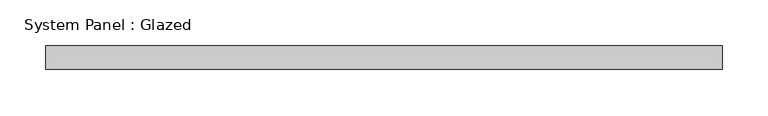
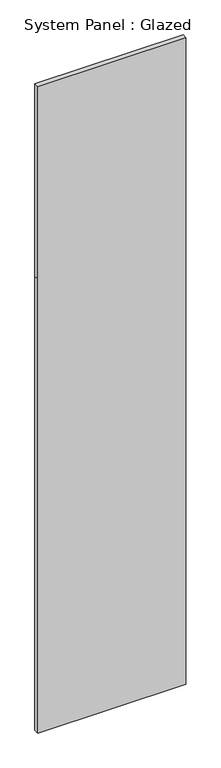
"""IFC4 building model written with IfcOpenShell, lengths in millimetres: plate geometry, System Panel : Glazed."""

import ifcopenshell
import ifcopenshell.guid

model = None  # the IFC model being written
_history = None  # IfcOwnerHistory: only IFC2X3 demands one
_inside = {}  # id of a spatial element -> (the spatial element, [elements in it])
_under = {}  # id of a project, library or spatial element -> (it, [spatial elements below it])
_declared = {}  # id of a project -> (the project, [libraries it declares])
_typed = {}  # id of a type object -> (the type object, [elements of that type])
_made_of = {}  # id of a material, layer set ... -> (it, [elements and type objects made of it])


def new_model(schema):
    """Start an empty IFC model of exactly this schema.

    Asked for "IFC4X3", IfcOpenShell would pick the latest addendum, in which some entities
    have other attributes; the version numbers below select the first issue.
    IFC2X3 requires an IfcOwnerHistory on every rooted entity: one is made here for all.
    """
    global model, _history
    if schema == "IFC4X3":
        model = ifcopenshell.file(schema_version=(4, 3, 0, 0))
    else:
        model = ifcopenshell.file(schema=schema)
    _inside.clear()
    _under.clear()
    _declared.clear()
    _typed.clear()
    _made_of.clear()
    _history = None
    if model.schema == "IFC2X3":
        org = make("IfcOrganization", Name="unknown")
        user = make(
            "IfcPersonAndOrganization",
            ThePerson=make("IfcPerson", FamilyName="unknown"),
            TheOrganization=org,
        )
        app = make(
            "IfcApplication",
            ApplicationDeveloper=org,
            Version="unknown",
            ApplicationFullName="unknown",
            ApplicationIdentifier="unknown",
        )
        _history = make(
            "IfcOwnerHistory",
            OwningUser=user,
            OwningApplication=app,
            ChangeAction="ADDED",
            CreationDate=0,
        )
    return model


def make(cls, **values):
    """One entity of the class cls with the attributes given. An attribute that is None is left unset."""
    return model.create_entity(
        cls, **{name: value for name, value in values.items() if value is not None}
    )


def rooted(cls, **values):
    """An entity with a GlobalId (a new one), such as an element, a storey or a relation."""
    return make(cls, GlobalId=ifcopenshell.guid.new(), OwnerHistory=_history, **values)


def si_unit(unit_type, name, prefix=None):
    """IfcSIUnit, for example si_unit("LENGTHUNIT", "METRE", prefix="MILLI")."""
    return make("IfcSIUnit", UnitType=unit_type, Prefix=prefix, Name=name)


def assignment(units):
    """IfcUnitAssignment: the units of a project."""
    return None if units is None else make("IfcUnitAssignment", Units=units)


def point(xyz):
    """IfcCartesianPoint."""
    return None if xyz is None else make("IfcCartesianPoint", Coordinates=xyz)


def direction(xyz):
    """IfcDirection."""
    return None if xyz is None else make("IfcDirection", DirectionRatios=xyz)


def frame(location, z_axis=None, x_axis=None):
    """IfcAxis2Placement3D, a coordinate frame: its origin and axes. An axis left out is left unset."""
    return make(
        "IfcAxis2Placement3D",
        Location=point(location),
        Axis=direction(z_axis),
        RefDirection=direction(x_axis),
    )


def origin():
    """The frame at (0, 0, 0) with its axes left unset."""
    return frame((0.0, 0.0, 0.0))


def place(relative_to, where):
    """IfcLocalPlacement: puts the frame where relative to a parent placement (None: the world)."""
    return make(
        "IfcLocalPlacement", PlacementRelTo=relative_to, RelativePlacement=where
    )


def context(
    kind, dimensions, precision=None, world=None, true_north=None, identifier=None
):
    """IfcGeometricRepresentationContext, for example the 3D "Model" context."""
    return make(
        "IfcGeometricRepresentationContext",
        ContextIdentifier=identifier,
        ContextType=kind,
        CoordinateSpaceDimension=dimensions,
        Precision=precision,
        WorldCoordinateSystem=world,
        TrueNorth=true_north,
    )


def project(units=None, contexts=None):
    """IfcProject with its units and contexts."""
    return rooted(
        "IfcProject",
        Name="project",
        RepresentationContexts=contexts,
        UnitsInContext=assignment(units),
    )


def spatial(cls, under=None, at=None, **own):
    """A site, building, storey or space (cls), placed at a placement, below another one or the project."""
    s = rooted(cls, ObjectPlacement=at, **own)
    if under is not None:
        _under.setdefault(under.id(), (under, []))[1].append(s)
    return s


def polyline(points):
    """IfcPolyline through the points."""
    return make("IfcPolyline", Points=[point(p) for p in points])


def outline(outer, holes=None, kind="AREA"):
    """IfcArbitraryClosedProfileDef: a profile drawn as a closed curve; with holes, ...WithVoids."""
    if holes is None:
        return make("IfcArbitraryClosedProfileDef", ProfileType=kind, OuterCurve=outer)
    return make(
        "IfcArbitraryProfileDefWithVoids",
        ProfileType=kind,
        OuterCurve=outer,
        InnerCurves=holes,
    )


def extrude(swept, where, along, depth):
    """IfcExtrudedAreaSolid: the profile swept, set in the frame where, extruded along a direction by depth."""
    return make(
        "IfcExtrudedAreaSolid",
        SweptArea=swept,
        Position=where,
        ExtrudedDirection=direction(along),
        Depth=depth,
    )


def shape(context_of_items, identifier, shape_type, items):
    """IfcShapeRepresentation: the items that make up one representation, for example the "Body"."""
    return make(
        "IfcShapeRepresentation",
        ContextOfItems=context_of_items,
        RepresentationIdentifier=identifier,
        RepresentationType=shape_type,
        Items=items,
    )


def source(mapping_origin, context_of_items, identifier, shape_type, items):
    """IfcRepresentationMap: a shape defined once, which mapped items show again and again."""
    return make(
        "IfcRepresentationMap",
        MappingOrigin=mapping_origin,
        MappedRepresentation=shape(context_of_items, identifier, shape_type, items),
    )


def transform(
    local_origin,
    x_axis=None,
    y_axis=None,
    z_axis=None,
    scale=None,
    scale2=None,
    scale3=None,
    uniform=True,
):
    """IfcCartesianTransformationOperator3D, or its non-uniform kind. x_axis, y_axis, z_axis: its Axis1, 2, 3."""
    if uniform:
        return make(
            "IfcCartesianTransformationOperator3D",
            Axis1=direction(x_axis),
            Axis2=direction(y_axis),
            LocalOrigin=point(local_origin),
            Scale=scale,
            Axis3=direction(z_axis),
        )
    return make(
        "IfcCartesianTransformationOperator3DnonUniform",
        Axis1=direction(x_axis),
        Axis2=direction(y_axis),
        LocalOrigin=point(local_origin),
        Scale=scale,
        Axis3=direction(z_axis),
        Scale2=scale2,
        Scale3=scale3,
    )


def mapped(mapping_source, mapping_target):
    """IfcMappedItem: shows the shape of a source again, moved by a transform."""
    return make(
        "IfcMappedItem", MappingSource=mapping_source, MappingTarget=mapping_target
    )


def made_of(thing, what):
    """Note that an element or type object is made of a material, layer set ...; save() writes the relation."""
    if what is not None:
        _made_of.setdefault(what.id(), (what, []))[1].append(thing)
    return thing


def element(
    cls,
    number,
    at=None,
    inside=None,
    cuts=None,
    type_object=None,
    material=None,
    context=None,
    identifier="Body",
    shape_type=None,
    held_by="IfcProductDefinitionShape",
    body=None,
    shapes=None,
    **own,
):
    """One element of the class cls, such as IfcWall. Its Tag is "e" and its number.

    at: its placement. inside: the storey or other place that contains it. cuts: it is an
    opening in that element (IfcRelVoidsElement). A single representation is given by context,
    identifier, shape_type and body (its items); several are given by shapes. held_by: the class
    of the entity that holds the representations. save() writes the other relations.
    """
    e = rooted(cls, Tag="e%d" % number, ObjectPlacement=at, **own)
    if body is not None:
        shapes = [shape(context, identifier, shape_type, body)]
    if shapes is not None:
        e.Representation = make(held_by, Representations=shapes)
    if inside is not None:
        _inside.setdefault(inside.id(), (inside, []))[1].append(e)
    if cuts is not None:
        rooted(
            "IfcRelVoidsElement", RelatingBuildingElement=cuts, RelatedOpeningElement=e
        )
    if type_object is not None:
        _typed.setdefault(type_object.id(), (type_object, []))[1].append(e)
    return made_of(e, material)


def aggregate(whole, parts):
    """IfcRelAggregates: a whole, such as a stair, and the parts it consists of."""
    return rooted("IfcRelAggregates", RelatingObject=whole, RelatedObjects=parts)


def save(model, path):
    """Write the relations noted so far, then the file.

    IfcRelAggregates (storeys below a building ...), IfcRelContainedInSpatialStructure (elements
    in a storey), IfcRelDefinesByType, IfcRelAssociatesMaterial and IfcRelDeclares: one each for
    every whole, place, type object, material and project.
    """
    for whole, parts in _under.values():
        aggregate(whole, parts)
    for where, things in _inside.values():
        rooted(
            "IfcRelContainedInSpatialStructure",
            RelatedElements=things,
            RelatingStructure=where,
        )
    for kind, things in _typed.values():
        rooted("IfcRelDefinesByType", RelatedObjects=things, RelatingType=kind)
    for what, things in _made_of.values():
        rooted("IfcRelAssociatesMaterial", RelatedObjects=things, RelatingMaterial=what)
    for by, libraries in _declared.values():
        rooted("IfcRelDeclares", RelatingContext=by, RelatedDefinitions=libraries)
    model.write(path)


def system_panel_glazed_b9d338b1(model_context):
    return source(origin(), model_context, "Body", "SweptSolid", [
        extrude(outline(polyline([(0.0, -368.3), (0.0, 368.3), (2387.6, 368.3), (3397.25, 368.3), (3397.25, -368.3), (2387.6, -368.3), (0.0, -368.3)])), frame((0.0, -31.75, 0.0), z_axis=(0.0, 1.0, 0.0), x_axis=(0.0, 0.0, 1.0)), (0.0, 0.0, 1.0), 25.4),
    ])


if __name__ == "__main__":
    model = new_model("IFC4")
    model_context = context("Model", 3, world=origin())
    ifc_project = project(units=[si_unit("LENGTHUNIT", "METRE", prefix="MILLI")], contexts=[model_context])
    site = spatial("IfcSite", under=ifc_project)
    building = spatial("IfcBuilding", under=site)
    placement = place(None, origin())
    system_panel_glazed_shape = system_panel_glazed_b9d338b1(model_context)
    element("IfcPlate", 1, ObjectType="System Panel : Glazed", at=placement, inside=building, context=model_context, shape_type="MappedRepresentation", body=[
        mapped(system_panel_glazed_shape, transform((0.0, 0.0, 0.0), x_axis=(1.0, 0.0, 0.0), y_axis=(0.0, 1.0, 0.0), z_axis=(0.0, 0.0, 1.0))),
    ])
    save(model, "model.ifc")

# Revit data of these elements
# Type "System Panel : Glazed"
#   Construction Type Id = "GSP4R"
#   Analytic Construction = "1/8 in Pilkington single glazing"
#   Visual Light Transmittance = 0.9
#   Solar Heat Gain Coefficient = 0.86
#   Heat Transfer Coefficient (U) = 6.7069 W/(m²·K)
#   Elevation_Transparency_Hack = 70
# Element 1 (IfcPlate, "System Panel : Glazed")
#   Materials on its faces: "Glass"
# Materials
#   "Glass": class "Glass", colour RGB 0 128 192, transparency 0.75, Description = "Soda Lime Glass", Cost = 0
